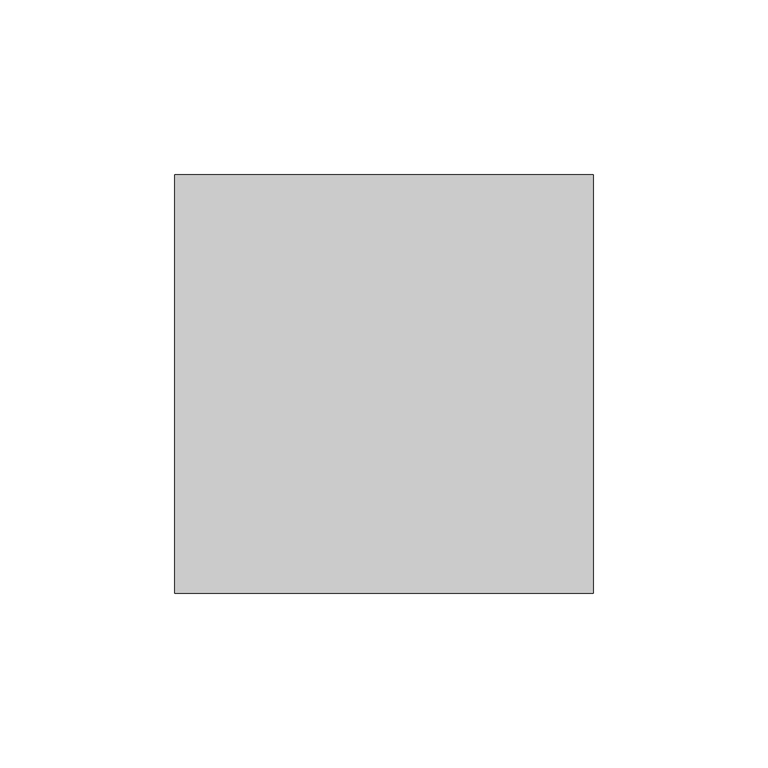
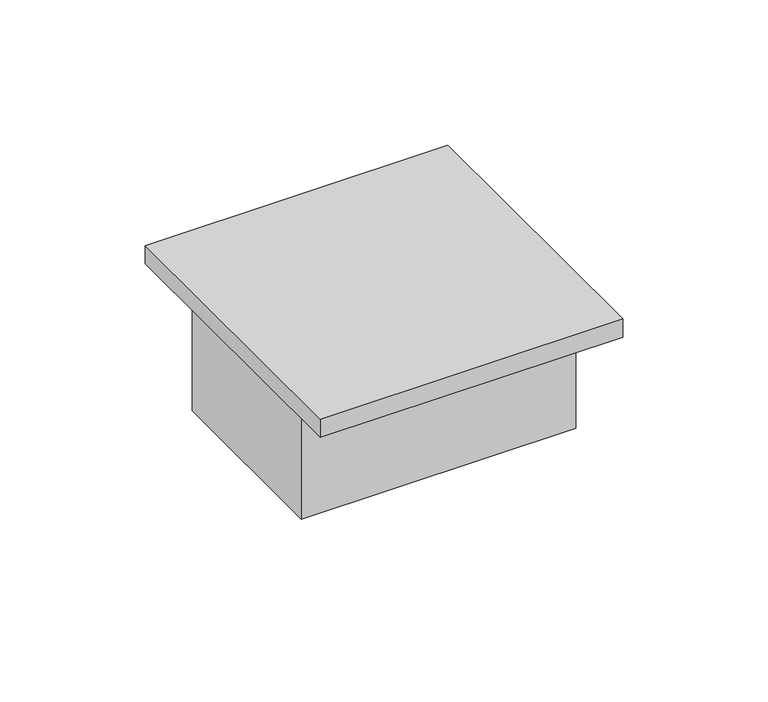
"""IFC4 building model written with IfcOpenShell, lengths in millimetres: proxy geometry, 262726-JBOX : JBox."""

from ifc_helpers import new_model, si_unit, frame, origin, origin_with_axes, place, context, project, spatial, polyline, outline, extrude, source, transform, mapped, element, save


def electrical_fixtures_317c45e1(model_context):
    return source(origin(), model_context, "Body", "SweptSolid", [
        extrude(outline(polyline([(38.375, 60.0), (38.375, -60.0), (-81.625, -60.0), (-81.625, 60.0), (38.375, 60.0)])), origin_with_axes(), (0.0, 0.0, 1.0), 7.6398437),
        extrude(outline(polyline([(32.875, 37.5), (32.875, -37.5), (-76.125, -37.5), (-76.125, 37.5), (32.875, 37.5)])), frame((0.0, 0.0, -50.0), z_axis=(0.0, 0.0, 1.0), x_axis=(1.0, 0.0, 0.0)), (0.0, 0.0, 1.0), 50.0),
    ])


if __name__ == "__main__":
    model = new_model("IFC4")
    model_context = context("Model", 3, world=origin())
    ifc_project = project(units=[si_unit("LENGTHUNIT", "METRE", prefix="MILLI")], contexts=[model_context])
    site = spatial("IfcSite", under=ifc_project)
    building = spatial("IfcBuilding", under=site)
    placement = place(None, origin())
    electrical_fixtures_shape = electrical_fixtures_317c45e1(model_context)
    element("IfcBuildingElementProxy", 1, Name="262726-JBOX : JBox", ObjectType="262726-JBOX : JBox", at=placement, inside=building, context=model_context, shape_type="MappedRepresentation", body=[
        mapped(electrical_fixtures_shape, transform((0.0, 0.0, 0.0), x_axis=(1.0, 0.0, 0.0), y_axis=(0.0, 1.0, 0.0), z_axis=(0.0, 0.0, 1.0))),
    ])
    save(model, "model.ifc")

# Revit data of these elements
# Type "262726-JBOX : JBox"
#   MasterFormat = "26 27 26 Wiring Devices"
#   Model = "Generic"
#   Manufacturer = "Generic"
#   Label = "2400"
#   Description = "JUNCTION BOX"
#   Voltage [instance default] = 230 V
#   Power Factor [instance default] = 1
#   Phase = 1
#   Frequency = 50 Hz
#   Default Elevation = 2400 mm
#   Cost = 4
#   Apparent Load [instance default] = 180 VA
#   Number of Poles [instance default] = 1
#   Anno Adjust [instance default] = no
#   Symbol = SYMBOL-Electrical : Junction Box
#   Load Classification = HVAC
#   Face Plate = element 489477
#   Assembly Code = ""
# Element 1 (IfcBuildingElementProxy, "262726-JBOX : JBox")
#   Voltage = 240 V
#   Apparent Load = 2000 VA
#   Number of Poles = 2
